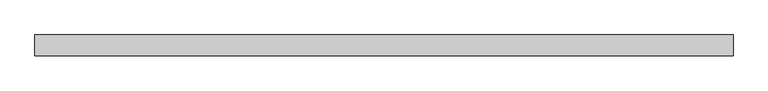
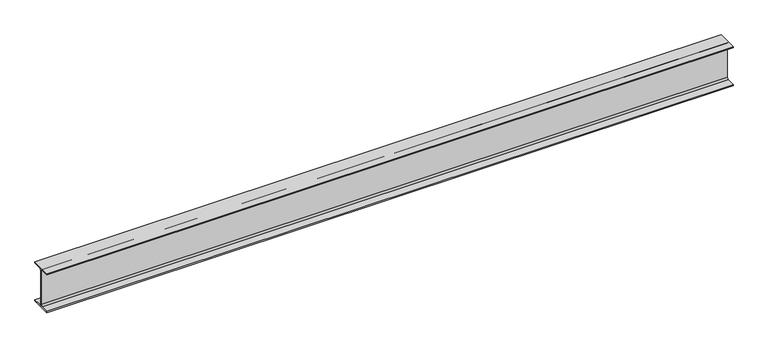
"""IFC4 building model written with IfcOpenShell, lengths in millimetres: beam geometry, 0912_Steel Framing_H-KSD3502 : H_SB_ASB_H-350x175x7x11."""

import ifcopenshell
import ifcopenshell.guid

model = None  # the IFC model being written
_history = None  # IfcOwnerHistory: only IFC2X3 demands one
_inside = {}  # id of a spatial element -> (the spatial element, [elements in it])
_under = {}  # id of a project, library or spatial element -> (it, [spatial elements below it])
_declared = {}  # id of a project -> (the project, [libraries it declares])
_typed = {}  # id of a type object -> (the type object, [elements of that type])
_made_of = {}  # id of a material, layer set ... -> (it, [elements and type objects made of it])


def new_model(schema):
    """Start an empty IFC model of exactly this schema.

    Asked for "IFC4X3", IfcOpenShell would pick the latest addendum, in which some entities
    have other attributes; the version numbers below select the first issue.
    IFC2X3 requires an IfcOwnerHistory on every rooted entity: one is made here for all.
    """
    global model, _history
    if schema == "IFC4X3":
        model = ifcopenshell.file(schema_version=(4, 3, 0, 0))
    else:
        model = ifcopenshell.file(schema=schema)
    _inside.clear()
    _under.clear()
    _declared.clear()
    _typed.clear()
    _made_of.clear()
    _history = None
    if model.schema == "IFC2X3":
        org = make("IfcOrganization", Name="unknown")
        user = make(
            "IfcPersonAndOrganization",
            ThePerson=make("IfcPerson", FamilyName="unknown"),
            TheOrganization=org,
        )
        app = make(
            "IfcApplication",
            ApplicationDeveloper=org,
            Version="unknown",
            ApplicationFullName="unknown",
            ApplicationIdentifier="unknown",
        )
        _history = make(
            "IfcOwnerHistory",
            OwningUser=user,
            OwningApplication=app,
            ChangeAction="ADDED",
            CreationDate=0,
        )
    return model


def make(cls, **values):
    """One entity of the class cls with the attributes given. An attribute that is None is left unset."""
    return model.create_entity(
        cls, **{name: value for name, value in values.items() if value is not None}
    )


def rooted(cls, **values):
    """An entity with a GlobalId (a new one), such as an element, a storey or a relation."""
    return make(cls, GlobalId=ifcopenshell.guid.new(), OwnerHistory=_history, **values)


def si_unit(unit_type, name, prefix=None):
    """IfcSIUnit, for example si_unit("LENGTHUNIT", "METRE", prefix="MILLI")."""
    return make("IfcSIUnit", UnitType=unit_type, Prefix=prefix, Name=name)


def assignment(units):
    """IfcUnitAssignment: the units of a project."""
    return None if units is None else make("IfcUnitAssignment", Units=units)


def point(xyz):
    """IfcCartesianPoint."""
    return None if xyz is None else make("IfcCartesianPoint", Coordinates=xyz)


def direction(xyz):
    """IfcDirection."""
    return None if xyz is None else make("IfcDirection", DirectionRatios=xyz)


def frame(location, z_axis=None, x_axis=None):
    """IfcAxis2Placement3D, a coordinate frame: its origin and axes. An axis left out is left unset."""
    return make(
        "IfcAxis2Placement3D",
        Location=point(location),
        Axis=direction(z_axis),
        RefDirection=direction(x_axis),
    )


def frame_2d(location, x_axis=None):
    """IfcAxis2Placement2D, a coordinate frame in the plane: its origin and x axis."""
    return make(
        "IfcAxis2Placement2D", Location=point(location), RefDirection=direction(x_axis)
    )


def origin():
    """The frame at (0, 0, 0) with its axes left unset."""
    return frame((0.0, 0.0, 0.0))


def place(relative_to, where):
    """IfcLocalPlacement: puts the frame where relative to a parent placement (None: the world)."""
    return make(
        "IfcLocalPlacement", PlacementRelTo=relative_to, RelativePlacement=where
    )


def context(
    kind, dimensions, precision=None, world=None, true_north=None, identifier=None
):
    """IfcGeometricRepresentationContext, for example the 3D "Model" context."""
    return make(
        "IfcGeometricRepresentationContext",
        ContextIdentifier=identifier,
        ContextType=kind,
        CoordinateSpaceDimension=dimensions,
        Precision=precision,
        WorldCoordinateSystem=world,
        TrueNorth=true_north,
    )


def project(units=None, contexts=None):
    """IfcProject with its units and contexts."""
    return rooted(
        "IfcProject",
        Name="project",
        RepresentationContexts=contexts,
        UnitsInContext=assignment(units),
    )


def spatial(cls, under=None, at=None, **own):
    """A site, building, storey or space (cls), placed at a placement, below another one or the project."""
    s = rooted(cls, ObjectPlacement=at, **own)
    if under is not None:
        _under.setdefault(under.id(), (under, []))[1].append(s)
    return s


def polyline(points):
    """IfcPolyline through the points."""
    return make("IfcPolyline", Points=[point(p) for p in points])


def circle_curve(where, radius):
    """IfcCircle in the frame where."""
    return make("IfcCircle", Position=where, Radius=radius)


def trimmed(basis, trim1, trim2, sense, master):
    """IfcTrimmedCurve: the piece of a basis curve between two trims."""
    return make(
        "IfcTrimmedCurve",
        BasisCurve=basis,
        Trim1=trim1,
        Trim2=trim2,
        SenseAgreement=sense,
        MasterRepresentation=master,
    )


def segment(curve, same_sense, transition):
    """IfcCompositeCurveSegment."""
    return make(
        "IfcCompositeCurveSegment",
        Transition=transition,
        SameSense=same_sense,
        ParentCurve=curve,
    )


def composite_curve(segments, self_intersect=None):
    """IfcCompositeCurve: segments joined end to end."""
    return make("IfcCompositeCurve", Segments=segments, SelfIntersect=self_intersect)


def outline(outer, holes=None, kind="AREA"):
    """IfcArbitraryClosedProfileDef: a profile drawn as a closed curve; with holes, ...WithVoids."""
    if holes is None:
        return make("IfcArbitraryClosedProfileDef", ProfileType=kind, OuterCurve=outer)
    return make(
        "IfcArbitraryProfileDefWithVoids",
        ProfileType=kind,
        OuterCurve=outer,
        InnerCurves=holes,
    )


def extrude(swept, where, along, depth):
    """IfcExtrudedAreaSolid: the profile swept, set in the frame where, extruded along a direction by depth."""
    return make(
        "IfcExtrudedAreaSolid",
        SweptArea=swept,
        Position=where,
        ExtrudedDirection=direction(along),
        Depth=depth,
    )


def shape(context_of_items, identifier, shape_type, items):
    """IfcShapeRepresentation: the items that make up one representation, for example the "Body"."""
    return make(
        "IfcShapeRepresentation",
        ContextOfItems=context_of_items,
        RepresentationIdentifier=identifier,
        RepresentationType=shape_type,
        Items=items,
    )


def source(mapping_origin, context_of_items, identifier, shape_type, items):
    """IfcRepresentationMap: a shape defined once, which mapped items show again and again."""
    return make(
        "IfcRepresentationMap",
        MappingOrigin=mapping_origin,
        MappedRepresentation=shape(context_of_items, identifier, shape_type, items),
    )


def transform(
    local_origin,
    x_axis=None,
    y_axis=None,
    z_axis=None,
    scale=None,
    scale2=None,
    scale3=None,
    uniform=True,
):
    """IfcCartesianTransformationOperator3D, or its non-uniform kind. x_axis, y_axis, z_axis: its Axis1, 2, 3."""
    if uniform:
        return make(
            "IfcCartesianTransformationOperator3D",
            Axis1=direction(x_axis),
            Axis2=direction(y_axis),
            LocalOrigin=point(local_origin),
            Scale=scale,
            Axis3=direction(z_axis),
        )
    return make(
        "IfcCartesianTransformationOperator3DnonUniform",
        Axis1=direction(x_axis),
        Axis2=direction(y_axis),
        LocalOrigin=point(local_origin),
        Scale=scale,
        Axis3=direction(z_axis),
        Scale2=scale2,
        Scale3=scale3,
    )


def mapped(mapping_source, mapping_target):
    """IfcMappedItem: shows the shape of a source again, moved by a transform."""
    return make(
        "IfcMappedItem", MappingSource=mapping_source, MappingTarget=mapping_target
    )


def made_of(thing, what):
    """Note that an element or type object is made of a material, layer set ...; save() writes the relation."""
    if what is not None:
        _made_of.setdefault(what.id(), (what, []))[1].append(thing)
    return thing


def element(
    cls,
    number,
    at=None,
    inside=None,
    cuts=None,
    type_object=None,
    material=None,
    context=None,
    identifier="Body",
    shape_type=None,
    held_by="IfcProductDefinitionShape",
    body=None,
    shapes=None,
    **own,
):
    """One element of the class cls, such as IfcWall. Its Tag is "e" and its number.

    at: its placement. inside: the storey or other place that contains it. cuts: it is an
    opening in that element (IfcRelVoidsElement). A single representation is given by context,
    identifier, shape_type and body (its items); several are given by shapes. held_by: the class
    of the entity that holds the representations. save() writes the other relations.
    """
    e = rooted(cls, Tag="e%d" % number, ObjectPlacement=at, **own)
    if body is not None:
        shapes = [shape(context, identifier, shape_type, body)]
    if shapes is not None:
        e.Representation = make(held_by, Representations=shapes)
    if inside is not None:
        _inside.setdefault(inside.id(), (inside, []))[1].append(e)
    if cuts is not None:
        rooted(
            "IfcRelVoidsElement", RelatingBuildingElement=cuts, RelatedOpeningElement=e
        )
    if type_object is not None:
        _typed.setdefault(type_object.id(), (type_object, []))[1].append(e)
    return made_of(e, material)


def aggregate(whole, parts):
    """IfcRelAggregates: a whole, such as a stair, and the parts it consists of."""
    return rooted("IfcRelAggregates", RelatingObject=whole, RelatedObjects=parts)


def save(model, path):
    """Write the relations noted so far, then the file.

    IfcRelAggregates (storeys below a building ...), IfcRelContainedInSpatialStructure (elements
    in a storey), IfcRelDefinesByType, IfcRelAssociatesMaterial and IfcRelDeclares: one each for
    every whole, place, type object, material and project.
    """
    for whole, parts in _under.values():
        aggregate(whole, parts)
    for where, things in _inside.values():
        rooted(
            "IfcRelContainedInSpatialStructure",
            RelatedElements=things,
            RelatingStructure=where,
        )
    for kind, things in _typed.values():
        rooted("IfcRelDefinesByType", RelatedObjects=things, RelatingType=kind)
    for what, things in _made_of.values():
        rooted("IfcRelAssociatesMaterial", RelatedObjects=things, RelatingMaterial=what)
    for by, libraries in _declared.values():
        rooted("IfcRelDeclares", RelatingContext=by, RelatedDefinitions=libraries)
    model.write(path)


def beam_b071fafb(model_context):
    return source(origin(), model_context, "Body", "SweptSolid", [
        extrude(outline(composite_curve([segment(polyline([(87.5, -164.0), (87.5, -175.0), (-87.5, -175.0), (-87.5, -164.0), (-17.5, -164.0)]), True, "CONTINUOUS"), segment(trimmed(circle_curve(frame_2d((-17.5, -150.0)), 14.0), [point((-17.5, -164.0))], [point((-3.5, -150.0))], True, "CARTESIAN"), True, "CONTINUOUS"), segment(polyline([(-3.5, -150.0), (-3.5, 150.0)]), True, "CONTINUOUS"), segment(trimmed(circle_curve(frame_2d((-17.5, 150.0)), 14.0), [point((-3.5, 150.0))], [point((-17.5, 164.0))], True, "CARTESIAN"), True, "CONTINUOUS"), segment(polyline([(-17.5, 164.0), (-87.5, 164.0), (-87.5, 175.0), (87.5, 175.0), (87.5, 164.0), (17.5, 164.0)]), True, "CONTINUOUS"), segment(trimmed(circle_curve(frame_2d((17.5, 150.0)), 14.0), [point((17.5, 164.0))], [point((3.5, 150.0))], True, "CARTESIAN"), True, "CONTINUOUS"), segment(polyline([(3.5, 150.0), (3.5, -150.0)]), True, "CONTINUOUS"), segment(trimmed(circle_curve(frame_2d((17.5, -150.0)), 14.0), [point((3.5, -150.0))], [point((17.5, -164.0))], True, "CARTESIAN"), True, "CONTINUOUS"), segment(polyline([(17.5, -164.0), (87.5, -164.0)]), True, "CONTINUOUS")], self_intersect=False)), frame((-2920.1721181, 0.0, 0.0), z_axis=(1.0, 0.0, 0.0), x_axis=(0.0, 1.0, 0.0)), (0.0, 0.0, 1.0), 5810.1548079),
    ])


if __name__ == "__main__":
    model = new_model("IFC4")
    model_context = context("Model", 3, world=origin())
    ifc_project = project(units=[si_unit("LENGTHUNIT", "METRE", prefix="MILLI")], contexts=[model_context])
    site = spatial("IfcSite", under=ifc_project)
    building = spatial("IfcBuilding", under=site)
    placement = place(None, origin())
    beam_shape = beam_b071fafb(model_context)
    element("IfcBeam", 1, ObjectType="0912_Steel Framing_H-KSD3502 : H_SB_ASB_H-350x175x7x11", at=placement, inside=building, context=model_context, shape_type="MappedRepresentation", body=[
        mapped(beam_shape, transform((0.0, 0.0, 0.0), x_axis=(1.0, 0.0, 0.0), y_axis=(0.0, 1.0, 0.0), z_axis=(0.0, 0.0, 1.0))),
    ])
    save(model, "model.ifc")

# Revit data of these elements
# Type "0912_Steel Framing_H-KSD3502 : H_SB_ASB_H-350x175x7x11"
#   H_WM Code_1 = "S01AA002-00001 | Main Steel Structure Fabrication Work | Shelter/Building | Medium Steel - Standard (90KG/M>Weight≥30KG/M) | Material: (   )"
#   H_WM Code_2 = "S03AA028-00001 | Main Steel Structure Erection Work | Shelter/Building | Medium Steel (90KG/M>Weight≥30KG/M) | Material: (   )"
#   H_WM Code_3 = "S01AA010-00001 | Main Steel Structure Fabrication Work | Shelter/Building | Steel Painting/Coating | for Non-Fireproofed Steel Surface, Surface Preparation, Primer, Second & Final Coat | Material: (   )"
#   H_Q'ty Cal Type Tag = "SB-Q2"
#   Width = 17.5 cm
#   Web Thickness = 0.7 cm
#   Web Fillet = 1.4 cm
#   Warping Constant = 282000.0 cm⁶
#   W = 0
#   Torsional Moment of Inertia = 19.4042 cm⁴
#   Section Area = 63.14 cm²
#   Plastic Modulus weak axis = 174.0 cm³
#   Plastic Modulus strong axis = 868.0 cm³
#   Perimeter = 1.36 m²/m
#   Nominal Weight = 49.60 kgf/m
#   Moment of Inertia weak axis = 984.00 cm⁴
#   Moment of Inertia strong axis = 13600.00 cm⁴
#   Height = 35.0 cm
#   Flange Thickness = 1.1 cm
#   Elastic Modulus weak axis = 112.0 cm³
#   Elastic Modulus strong axis = 775.0 cm³
#   Centroid Vertical = 17.5 cm
#   Centroid Horizontal = 8.75 cm
#   Ix = 136000000
#   Length [instance default] = 1.5240 m
#   Zx = 868000
#   b = 0.1750 m
#   h = 0.3500 m
#   r = 0.0140 m
#   s = 0.0070 m
#   t = 0.0110 m
#   A = 0.006314 m²
#   Structural Material [instance default] = Steel, 45-345
#   Assembly Code = ""
# Element 1 (IfcBeam, "0912_Steel Framing_H-KSD3502 : H_SB_ASB_H-350x175x7x11")
#   Structural Material = none
# Materials
#   "Steel, 45-345": class "Metal", colour RGB 189 187 185, transparency 0, Description = "Steel 345 MPa", Cost = 0
